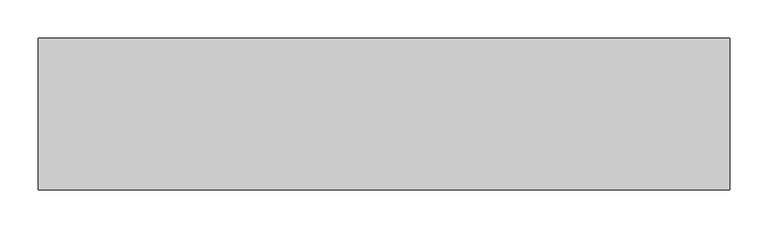
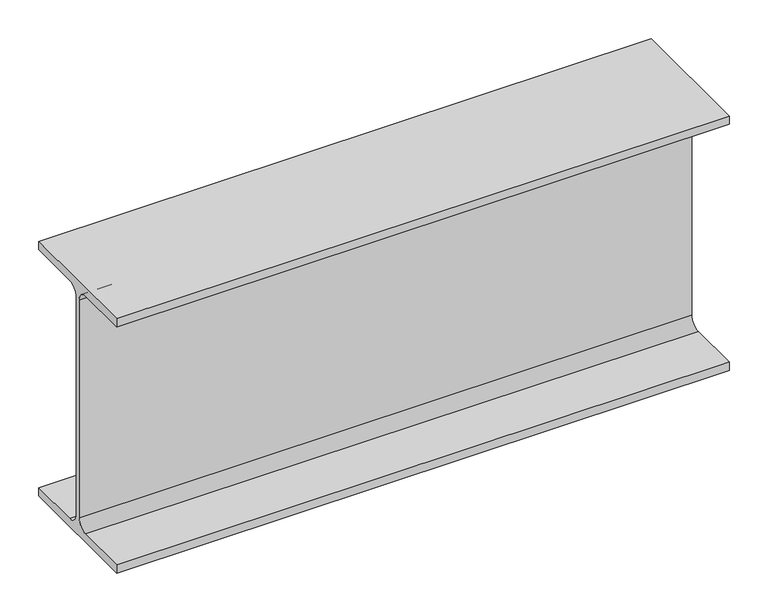
"""IFC4 building model written with IfcOpenShell, lengths in millimetres: beam geometry, Steel Framing_H_KS : H_SB_AR_S02_H-400x200x8x13_SCB1."""

import ifcopenshell
import ifcopenshell.guid

model = None  # the IFC model being written
_history = None  # IfcOwnerHistory: only IFC2X3 demands one
_inside = {}  # id of a spatial element -> (the spatial element, [elements in it])
_under = {}  # id of a project, library or spatial element -> (it, [spatial elements below it])
_declared = {}  # id of a project -> (the project, [libraries it declares])
_typed = {}  # id of a type object -> (the type object, [elements of that type])
_made_of = {}  # id of a material, layer set ... -> (it, [elements and type objects made of it])


def new_model(schema):
    """Start an empty IFC model of exactly this schema.

    Asked for "IFC4X3", IfcOpenShell would pick the latest addendum, in which some entities
    have other attributes; the version numbers below select the first issue.
    IFC2X3 requires an IfcOwnerHistory on every rooted entity: one is made here for all.
    """
    global model, _history
    if schema == "IFC4X3":
        model = ifcopenshell.file(schema_version=(4, 3, 0, 0))
    else:
        model = ifcopenshell.file(schema=schema)
    _inside.clear()
    _under.clear()
    _declared.clear()
    _typed.clear()
    _made_of.clear()
    _history = None
    if model.schema == "IFC2X3":
        org = make("IfcOrganization", Name="unknown")
        user = make(
            "IfcPersonAndOrganization",
            ThePerson=make("IfcPerson", FamilyName="unknown"),
            TheOrganization=org,
        )
        app = make(
            "IfcApplication",
            ApplicationDeveloper=org,
            Version="unknown",
            ApplicationFullName="unknown",
            ApplicationIdentifier="unknown",
        )
        _history = make(
            "IfcOwnerHistory",
            OwningUser=user,
            OwningApplication=app,
            ChangeAction="ADDED",
            CreationDate=0,
        )
    return model


def make(cls, **values):
    """One entity of the class cls with the attributes given. An attribute that is None is left unset."""
    return model.create_entity(
        cls, **{name: value for name, value in values.items() if value is not None}
    )


def rooted(cls, **values):
    """An entity with a GlobalId (a new one), such as an element, a storey or a relation."""
    return make(cls, GlobalId=ifcopenshell.guid.new(), OwnerHistory=_history, **values)


def si_unit(unit_type, name, prefix=None):
    """IfcSIUnit, for example si_unit("LENGTHUNIT", "METRE", prefix="MILLI")."""
    return make("IfcSIUnit", UnitType=unit_type, Prefix=prefix, Name=name)


def assignment(units):
    """IfcUnitAssignment: the units of a project."""
    return None if units is None else make("IfcUnitAssignment", Units=units)


def point(xyz):
    """IfcCartesianPoint."""
    return None if xyz is None else make("IfcCartesianPoint", Coordinates=xyz)


def direction(xyz):
    """IfcDirection."""
    return None if xyz is None else make("IfcDirection", DirectionRatios=xyz)


def frame(location, z_axis=None, x_axis=None):
    """IfcAxis2Placement3D, a coordinate frame: its origin and axes. An axis left out is left unset."""
    return make(
        "IfcAxis2Placement3D",
        Location=point(location),
        Axis=direction(z_axis),
        RefDirection=direction(x_axis),
    )


def frame_2d(location, x_axis=None):
    """IfcAxis2Placement2D, a coordinate frame in the plane: its origin and x axis."""
    return make(
        "IfcAxis2Placement2D", Location=point(location), RefDirection=direction(x_axis)
    )


def origin():
    """The frame at (0, 0, 0) with its axes left unset."""
    return frame((0.0, 0.0, 0.0))


def place(relative_to, where):
    """IfcLocalPlacement: puts the frame where relative to a parent placement (None: the world)."""
    return make(
        "IfcLocalPlacement", PlacementRelTo=relative_to, RelativePlacement=where
    )


def context(
    kind, dimensions, precision=None, world=None, true_north=None, identifier=None
):
    """IfcGeometricRepresentationContext, for example the 3D "Model" context."""
    return make(
        "IfcGeometricRepresentationContext",
        ContextIdentifier=identifier,
        ContextType=kind,
        CoordinateSpaceDimension=dimensions,
        Precision=precision,
        WorldCoordinateSystem=world,
        TrueNorth=true_north,
    )


def project(units=None, contexts=None):
    """IfcProject with its units and contexts."""
    return rooted(
        "IfcProject",
        Name="project",
        RepresentationContexts=contexts,
        UnitsInContext=assignment(units),
    )


def spatial(cls, under=None, at=None, **own):
    """A site, building, storey or space (cls), placed at a placement, below another one or the project."""
    s = rooted(cls, ObjectPlacement=at, **own)
    if under is not None:
        _under.setdefault(under.id(), (under, []))[1].append(s)
    return s


def polyline(points):
    """IfcPolyline through the points."""
    return make("IfcPolyline", Points=[point(p) for p in points])


def circle_curve(where, radius):
    """IfcCircle in the frame where."""
    return make("IfcCircle", Position=where, Radius=radius)


def trimmed(basis, trim1, trim2, sense, master):
    """IfcTrimmedCurve: the piece of a basis curve between two trims."""
    return make(
        "IfcTrimmedCurve",
        BasisCurve=basis,
        Trim1=trim1,
        Trim2=trim2,
        SenseAgreement=sense,
        MasterRepresentation=master,
    )


def segment(curve, same_sense, transition):
    """IfcCompositeCurveSegment."""
    return make(
        "IfcCompositeCurveSegment",
        Transition=transition,
        SameSense=same_sense,
        ParentCurve=curve,
    )


def composite_curve(segments, self_intersect=None):
    """IfcCompositeCurve: segments joined end to end."""
    return make("IfcCompositeCurve", Segments=segments, SelfIntersect=self_intersect)


def outline(outer, holes=None, kind="AREA"):
    """IfcArbitraryClosedProfileDef: a profile drawn as a closed curve; with holes, ...WithVoids."""
    if holes is None:
        return make("IfcArbitraryClosedProfileDef", ProfileType=kind, OuterCurve=outer)
    return make(
        "IfcArbitraryProfileDefWithVoids",
        ProfileType=kind,
        OuterCurve=outer,
        InnerCurves=holes,
    )


def extrude(swept, where, along, depth):
    """IfcExtrudedAreaSolid: the profile swept, set in the frame where, extruded along a direction by depth."""
    return make(
        "IfcExtrudedAreaSolid",
        SweptArea=swept,
        Position=where,
        ExtrudedDirection=direction(along),
        Depth=depth,
    )


def shape(context_of_items, identifier, shape_type, items):
    """IfcShapeRepresentation: the items that make up one representation, for example the "Body"."""
    return make(
        "IfcShapeRepresentation",
        ContextOfItems=context_of_items,
        RepresentationIdentifier=identifier,
        RepresentationType=shape_type,
        Items=items,
    )


def source(mapping_origin, context_of_items, identifier, shape_type, items):
    """IfcRepresentationMap: a shape defined once, which mapped items show again and again."""
    return make(
        "IfcRepresentationMap",
        MappingOrigin=mapping_origin,
        MappedRepresentation=shape(context_of_items, identifier, shape_type, items),
    )


def transform(
    local_origin,
    x_axis=None,
    y_axis=None,
    z_axis=None,
    scale=None,
    scale2=None,
    scale3=None,
    uniform=True,
):
    """IfcCartesianTransformationOperator3D, or its non-uniform kind. x_axis, y_axis, z_axis: its Axis1, 2, 3."""
    if uniform:
        return make(
            "IfcCartesianTransformationOperator3D",
            Axis1=direction(x_axis),
            Axis2=direction(y_axis),
            LocalOrigin=point(local_origin),
            Scale=scale,
            Axis3=direction(z_axis),
        )
    return make(
        "IfcCartesianTransformationOperator3DnonUniform",
        Axis1=direction(x_axis),
        Axis2=direction(y_axis),
        LocalOrigin=point(local_origin),
        Scale=scale,
        Axis3=direction(z_axis),
        Scale2=scale2,
        Scale3=scale3,
    )


def mapped(mapping_source, mapping_target):
    """IfcMappedItem: shows the shape of a source again, moved by a transform."""
    return make(
        "IfcMappedItem", MappingSource=mapping_source, MappingTarget=mapping_target
    )


def made_of(thing, what):
    """Note that an element or type object is made of a material, layer set ...; save() writes the relation."""
    if what is not None:
        _made_of.setdefault(what.id(), (what, []))[1].append(thing)
    return thing


def element(
    cls,
    number,
    at=None,
    inside=None,
    cuts=None,
    type_object=None,
    material=None,
    context=None,
    identifier="Body",
    shape_type=None,
    held_by="IfcProductDefinitionShape",
    body=None,
    shapes=None,
    **own,
):
    """One element of the class cls, such as IfcWall. Its Tag is "e" and its number.

    at: its placement. inside: the storey or other place that contains it. cuts: it is an
    opening in that element (IfcRelVoidsElement). A single representation is given by context,
    identifier, shape_type and body (its items); several are given by shapes. held_by: the class
    of the entity that holds the representations. save() writes the other relations.
    """
    e = rooted(cls, Tag="e%d" % number, ObjectPlacement=at, **own)
    if body is not None:
        shapes = [shape(context, identifier, shape_type, body)]
    if shapes is not None:
        e.Representation = make(held_by, Representations=shapes)
    if inside is not None:
        _inside.setdefault(inside.id(), (inside, []))[1].append(e)
    if cuts is not None:
        rooted(
            "IfcRelVoidsElement", RelatingBuildingElement=cuts, RelatedOpeningElement=e
        )
    if type_object is not None:
        _typed.setdefault(type_object.id(), (type_object, []))[1].append(e)
    return made_of(e, material)


def aggregate(whole, parts):
    """IfcRelAggregates: a whole, such as a stair, and the parts it consists of."""
    return rooted("IfcRelAggregates", RelatingObject=whole, RelatedObjects=parts)


def save(model, path):
    """Write the relations noted so far, then the file.

    IfcRelAggregates (storeys below a building ...), IfcRelContainedInSpatialStructure (elements
    in a storey), IfcRelDefinesByType, IfcRelAssociatesMaterial and IfcRelDeclares: one each for
    every whole, place, type object, material and project.
    """
    for whole, parts in _under.values():
        aggregate(whole, parts)
    for where, things in _inside.values():
        rooted(
            "IfcRelContainedInSpatialStructure",
            RelatedElements=things,
            RelatingStructure=where,
        )
    for kind, things in _typed.values():
        rooted("IfcRelDefinesByType", RelatedObjects=things, RelatingType=kind)
    for what, things in _made_of.values():
        rooted("IfcRelAssociatesMaterial", RelatedObjects=things, RelatingMaterial=what)
    for by, libraries in _declared.values():
        rooted("IfcRelDeclares", RelatingContext=by, RelatedDefinitions=libraries)
    model.write(path)


def beam_cf9155bb(model_context):
    return source(origin(), model_context, "Body", "SweptSolid", [
        extrude(outline(composite_curve([segment(polyline([(100.0, -187.0), (100.0, -200.0), (-100.0, -200.0), (-100.0, -187.0), (-20.0, -187.0)]), True, "CONTINUOUS"), segment(trimmed(circle_curve(frame_2d((-20.0, -171.0)), 16.0), [point((-20.0, -187.0))], [point((-4.0, -171.0))], True, "CARTESIAN"), True, "CONTINUOUS"), segment(polyline([(-4.0, -171.0), (-4.0, 171.0)]), True, "CONTINUOUS"), segment(trimmed(circle_curve(frame_2d((-20.0, 171.0)), 16.0), [point((-4.0, 171.0))], [point((-20.0, 187.0))], True, "CARTESIAN"), True, "CONTINUOUS"), segment(polyline([(-20.0, 187.0), (-100.0, 187.0), (-100.0, 200.0), (100.0, 200.0), (100.0, 187.0), (20.0, 187.0)]), True, "CONTINUOUS"), segment(trimmed(circle_curve(frame_2d((20.0, 171.0)), 16.0), [point((20.0, 187.0))], [point((4.0, 171.0))], True, "CARTESIAN"), True, "CONTINUOUS"), segment(polyline([(4.0, 171.0), (4.0, -171.0)]), True, "CONTINUOUS"), segment(trimmed(circle_curve(frame_2d((20.0, -171.0)), 16.0), [point((4.0, -171.0))], [point((20.0, -187.0))], True, "CARTESIAN"), True, "CONTINUOUS"), segment(polyline([(20.0, -187.0), (100.0, -187.0)]), True, "CONTINUOUS")], self_intersect=False)), frame((-380.0, 0.0, 0.0), z_axis=(1.0, 0.0, 0.0), x_axis=(0.0, 1.0, 0.0)), (0.0, 0.0, 1.0), 910.0),
    ])


if __name__ == "__main__":
    model = new_model("IFC4")
    model_context = context("Model", 3, world=origin())
    ifc_project = project(units=[si_unit("LENGTHUNIT", "METRE", prefix="MILLI")], contexts=[model_context])
    site = spatial("IfcSite", under=ifc_project)
    building = spatial("IfcBuilding", under=site)
    placement = place(None, origin())
    beam_shape = beam_cf9155bb(model_context)
    element("IfcBeam", 1, ObjectType="Steel Framing_H_KS : H_SB_AR_S02_H-400x200x8x13_SCB1", at=placement, inside=building, context=model_context, shape_type="MappedRepresentation", body=[
        mapped(beam_shape, transform((0.0, 0.0, 0.0), x_axis=(1.0, 0.0, 0.0), y_axis=(0.0, 1.0, 0.0), z_axis=(0.0, 0.0, 1.0))),
    ])
    save(model, "model.ifc")

# Revit data of these elements
# Type "Steel Framing_H_KS : H_SB_AR_S02_H-400x200x8x13_SCB1"
#   Type Comments = "MAIN"
#   Type Mark = "SCB1"
#   H_SectionID = "H-400x200x8x13"
#   H_Ratio for Additional Steel Plate = 0.2
#   Width = 20.0 cm
#   Web Thickness = 0.8 cm
#   Web Fillet = 1.6 cm
#   Warping Constant = 649000.0 cm⁶
#   Torsional Moment of Inertia = 35.8981 cm⁴
#   Section Area = 84.12 cm²
#   Plastic Modulus weak axis = 268.0 cm³
#   Plastic Modulus strong axis = 1330.0 cm³
#   Perimeter = 1.56 m²/m
#   Nominal Weight = 66.00 kgf/m
#   Moment of Inertia weak axis = 1740.00 cm⁴
#   Moment of Inertia strong axis = 23700.00 cm⁴
#   Height = 40.0 cm
#   Flange Thickness = 1.3 cm
#   Elastic Modulus weak axis = 174.0 cm³
#   Elastic Modulus strong axis = 1190.0 cm³
#   Centroid Vertical = 20.0 cm
#   Centroid Horizontal = 10.0 cm
#   Bolt Spacing = 8.89 cm
#   Length [instance default] = 1500 mm
#   Structural Material [instance default] = Steel, 45-345
#   Section Name Key = ""
#   Assembly Code = ""
# Element 1 (IfcBeam, "Steel Framing_H_KS : H_SB_AR_S02_H-400x200x8x13_SCB1")
#   Materials on its faces: "Steel, 45-345"
# Materials
#   "Steel, 45-345": class "Metal", colour RGB 189 187 185, transparency 0, Description = "Steel 345 MPa", Cost = 0
